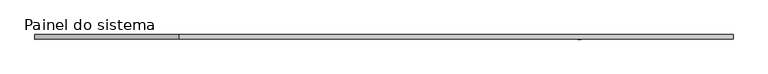
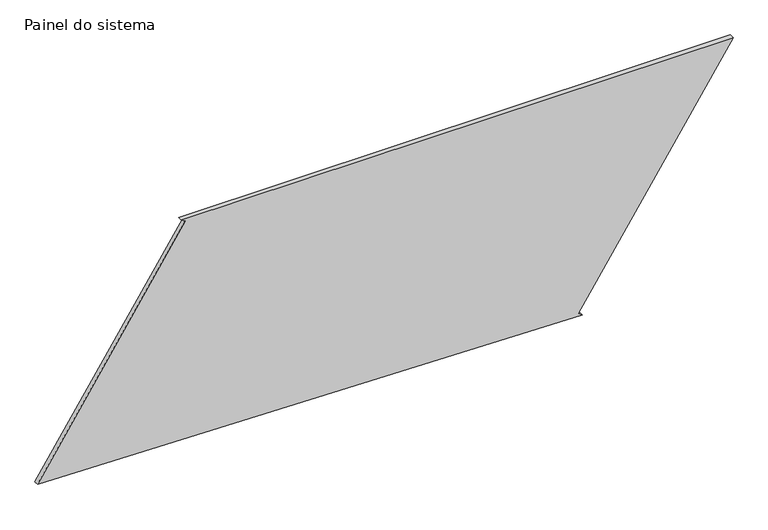
"""IFC4 building model written with IfcOpenShell, lengths in millimetres: plate geometry, Painel do sistema : Envidraçado."""

from ifc_helpers import new_model, si_unit, frame, origin, place, context, project, spatial, polyline, outline, extrude, source, transform, mapped, element, save


def painel_do_sistema_928481f9(model_context):
    return source(origin(), model_context, "Body", "SweptSolid", [
        extrude(outline(polyline([(0.0, 1083.5533146), (13.6354654, 1062.5992199), (1324.8284656, 1915.832303), (1324.8284656, -1123.7036194), (1311.1930002, -1102.7495247), (61.7003719, -1915.832303), (0.0, 1083.5533146)])), frame((0.0, 24.5, 0.0), z_axis=(0.0, 1.0, 0.0), x_axis=(0.0, 0.0, 1.0)), (0.0, 0.0, 1.0), 25.0),
    ])


if __name__ == "__main__":
    model = new_model("IFC4")
    model_context = context("Model", 3, world=origin())
    ifc_project = project(units=[si_unit("LENGTHUNIT", "METRE", prefix="MILLI")], contexts=[model_context])
    site = spatial("IfcSite", under=ifc_project)
    building = spatial("IfcBuilding", under=site)
    placement = place(None, origin())
    painel_do_sistema_shape = painel_do_sistema_928481f9(model_context)
    element("IfcPlate", 1, ObjectType="Painel do sistema : Envidraçado", at=placement, inside=building, context=model_context, shape_type="MappedRepresentation", body=[
        mapped(painel_do_sistema_shape, transform((0.0, 0.0, 0.0), x_axis=(1.0, 0.0, 0.0), y_axis=(0.0, 1.0, 0.0), z_axis=(0.0, 0.0, 1.0))),
    ])
    save(model, "model.ifc")

# Revit data of these elements
# Type "Painel do sistema : Envidraçado"
#   Construction Type Id = "GSP4R"
#   Analytic Construction = "Vidraça única Pilkington 1/8 pol"
#   Visual Light Transmittance = 0.9
#   Solar Heat Gain Coefficient = 0.86
#   Heat Transfer Coefficient (U) = 6.7069 W/(m²·K)
# Element 1 (IfcPlate, "Painel do sistema : Envidraçado")
#   Materials on its faces: "Vidro"
# Materials
#   "Vidro": class "Vidro", colour RGB 0 128 192, transparency 0.9, Description = "Vidro de sílica", Cost = 0
